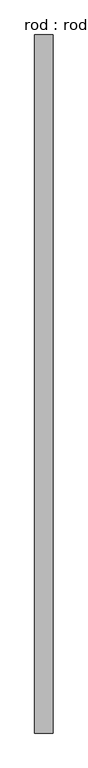
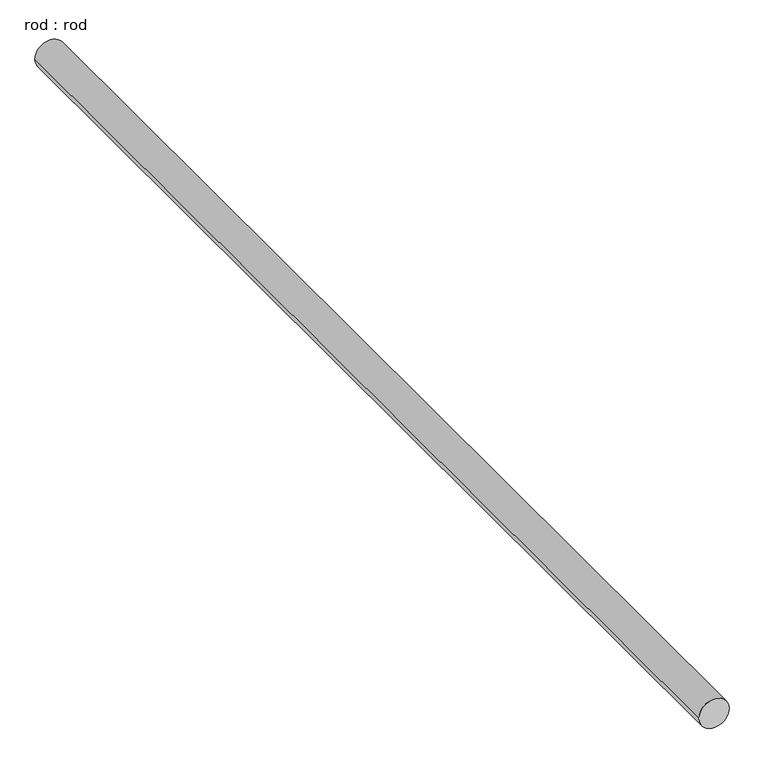
"""IFC4 building model written with IfcOpenShell, lengths in millimetres: proxy geometry, rod : rod."""

from ifc_helpers import new_model, si_unit, point, frame, frame_2d, origin, place, context, project, spatial, circle_curve, trimmed, segment, composite_curve, outline, extrude, source, transform, mapped, element, save


def rod_rod_aec4d1ff(model_context):
    return source(origin(), model_context, "Body", "SweptSolid", [
        extrude(outline(composite_curve([segment(trimmed(circle_curve(frame_2d((0.0108462, 0.0)), 200.0), [point((0.0108462, 200.0))], [point((0.0108462, -200.0))], False, "CARTESIAN"), True, "CONTINUOUS"), segment(trimmed(circle_curve(frame_2d((0.0108462, 0.0)), 200.0), [point((0.0108462, -200.0))], [point((0.0108462, 200.0))], False, "CARTESIAN"), True, "CONTINUOUS")], self_intersect=False)), frame((0.0, -3526.1332583, 0.0), z_axis=(0.0, 1.0, 0.0), x_axis=(0.0, 0.0, 1.0)), (0.0, 0.0, 1.0), 15237.7237473),
    ])


if __name__ == "__main__":
    model = new_model("IFC4")
    model_context = context("Model", 3, world=origin())
    ifc_project = project(units=[si_unit("LENGTHUNIT", "METRE", prefix="MILLI")], contexts=[model_context])
    site = spatial("IfcSite", under=ifc_project)
    building = spatial("IfcBuilding", under=site)
    placement = place(None, origin())
    rod_rod_shape = rod_rod_aec4d1ff(model_context)
    element("IfcBuildingElementProxy", 1, Name="rod : rod", ObjectType="rod : rod", at=placement, inside=building, context=model_context, shape_type="MappedRepresentation", body=[
        mapped(rod_rod_shape, transform((0.0, 0.0, 0.0), x_axis=(1.0, 0.0, 0.0), y_axis=(0.0, 1.0, 0.0), z_axis=(0.0, 0.0, 1.0))),
    ])
    save(model, "model.ifc")

# Revit data of these elements
# Type "rod : rod"
#   Default Elevation = 0
